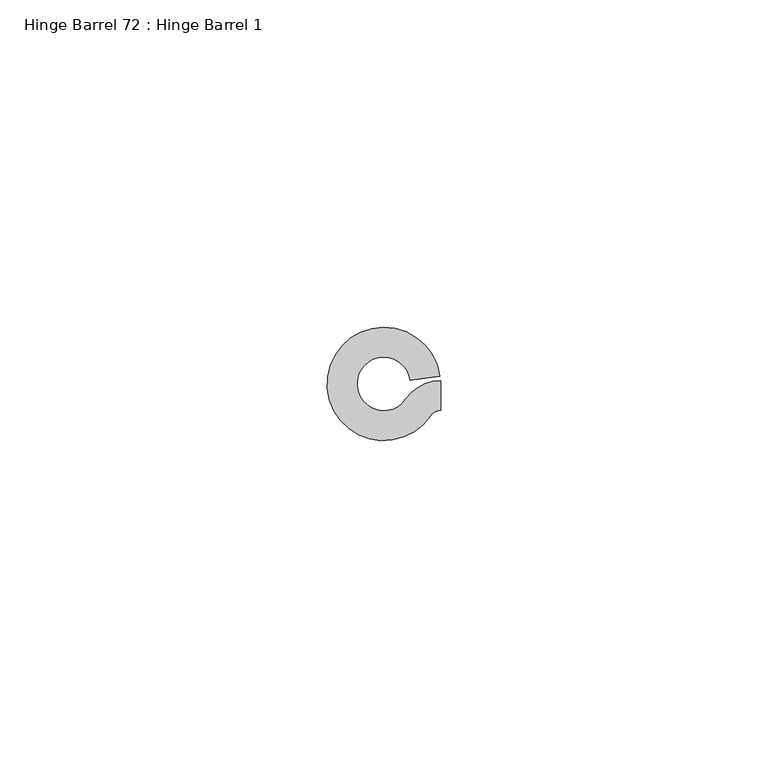
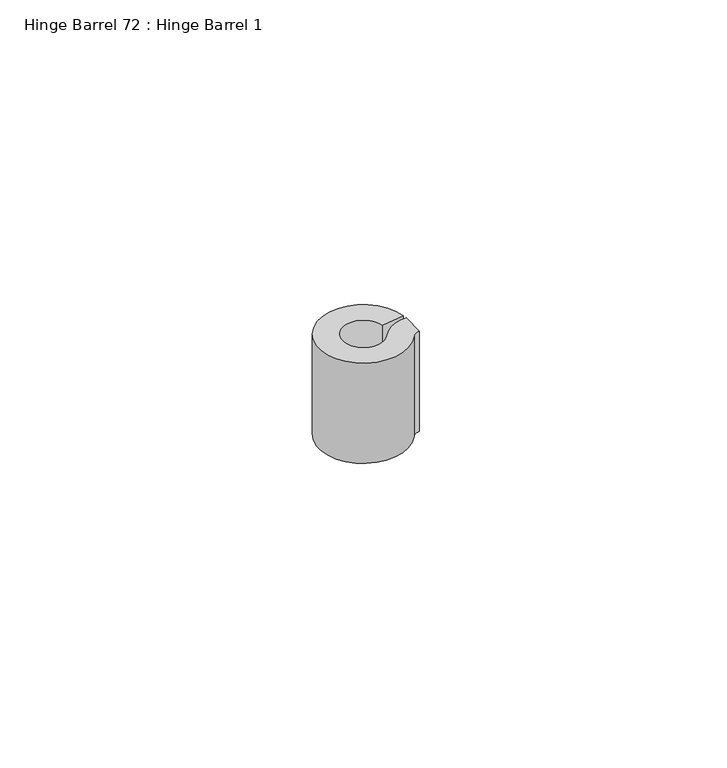
"""IFC4 building model written with IfcOpenShell, lengths in millimetres: proxy geometry, Hinge Barrel 72 : Hinge Barrel 1."""

from ifc_helpers import new_model, si_unit, point, frame, frame_2d, origin, place, context, project, spatial, polyline, circle_curve, trimmed, segment, composite_curve, outline, extrude, source, transform, mapped, element, save


def hinge_barrel_72_hinge_barrel_1_f5069254(model_context):
    return source(origin(), model_context, "Body", "SweptSolid", [
        extrude(outline(composite_curve([segment(trimmed(circle_curve(frame_2d((587327.8245257, -536316.2443067)), 6.4044851), [point((587322.5194669, -536312.6563017))], [point((587327.8245257, -536309.8398216))], False, "CARTESIAN"), True, "CONTINUOUS"), segment(polyline([(587327.8245257, -536309.8398216), (587327.8245257, -536314.4038841)]), True, "CONTINUOUS"), segment(trimmed(circle_curve(frame_2d((587327.8245257, -536316.2443067)), 1.8404226), [point((587327.8245257, -536314.4038841))], [point((587326.3000393, -536315.2132409))], True, "CARTESIAN"), True, "CONTINUOUS"), segment(trimmed(circle_curve(frame_2d((587319.1320739, -536310.3652841)), 8.6534625), [point((587326.3000393, -536315.2132409))], [point((587327.7022899, -536309.1678654))], False, "CARTESIAN"), True, "CONTINUOUS"), segment(polyline([(587327.7022899, -536309.1678654), (587323.1821338, -536309.7994153)]), True, "CONTINUOUS"), segment(trimmed(circle_curve(frame_2d((587319.1320739, -536310.3652841)), 4.0894), [point((587323.1821338, -536309.7994153))], [point((587322.5194669, -536312.6563017))], True, "CARTESIAN"), True, "CONTINUOUS")], self_intersect=False)), frame((0.0, 0.0, 1250.95), z_axis=(0.0, 0.0, 1.0), x_axis=(1.0, 0.0, 0.0)), (0.0, 0.0, 1.0), 20.8359375),
    ])


if __name__ == "__main__":
    model = new_model("IFC4")
    model_context = context("Model", 3, world=origin())
    ifc_project = project(units=[si_unit("LENGTHUNIT", "METRE", prefix="MILLI")], contexts=[model_context])
    site = spatial("IfcSite", under=ifc_project)
    building = spatial("IfcBuilding", under=site)
    placement = place(None, origin())
    hinge_barrel_72_hinge_barrel_1_shape = hinge_barrel_72_hinge_barrel_1_f5069254(model_context)
    element("IfcBuildingElementProxy", 1, Name="Hinge Barrel 72 : Hinge Barrel 1", ObjectType="Hinge Barrel 72 : Hinge Barrel 1", at=placement, inside=building, context=model_context, shape_type="MappedRepresentation", body=[
        mapped(hinge_barrel_72_hinge_barrel_1_shape, transform((0.0, 0.0, 0.0), x_axis=(1.0, 0.0, 0.0), y_axis=(0.0, 1.0, 0.0), z_axis=(0.0, 0.0, 1.0))),
    ])
    save(model, "model.ifc")

# Revit data of these elements
# Element 1 (IfcBuildingElementProxy, "Hinge Barrel 72 : Hinge Barrel 1")
#   Materials on its faces: "6\"X6\" WELD-ON STL BUTT HINGE"
# Materials
#   "6\"X6\" WELD-ON STL BUTT HINGE": class "Metal", colour RGB 189 187 185, transparency 0, Description = "Carbon steel", Cost = 0
